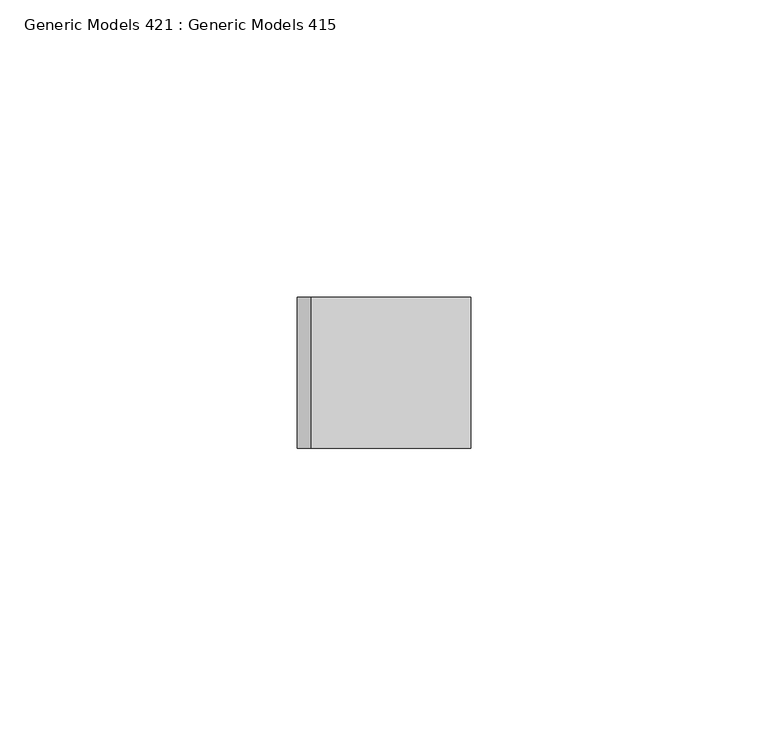
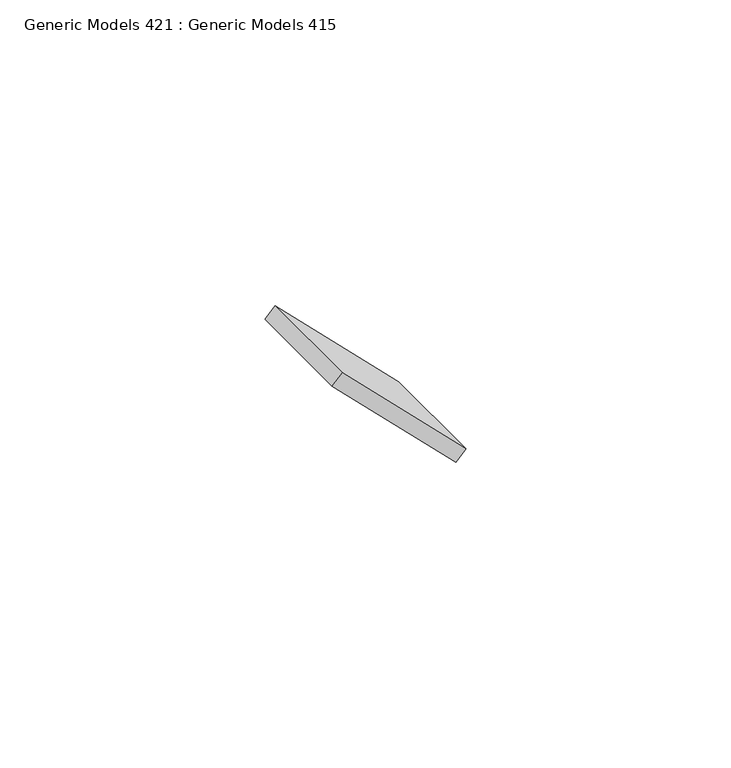
"""IFC4 building model written with IfcOpenShell, lengths in millimetres: proxy geometry, Generic Models 421 : Generic Models 415."""

from ifc_helpers import new_model, si_unit, frame, origin, place, context, project, spatial, polyline, outline, extrude, source, transform, mapped, element, save


def generic_models_421_generic_models_415_342b8473(model_context):
    return source(origin(), model_context, "Body", "SweptSolid", [
        extrude(outline(polyline([(0.0, -38.1), (0.0, 0.0), (25.4, 0.0), (25.4, -38.1), (0.0, -38.1)])), frame((-6869.8996186, -4475.9863946, 128607.0002957), z_axis=(0.7071067811864907, 0.0, 0.7071067811866044), x_axis=(0.0, -1.0, 0.0)), (0.0, 0.0, 1.0), 3.175),
    ])


if __name__ == "__main__":
    model = new_model("IFC4")
    model_context = context("Model", 3, world=origin())
    ifc_project = project(units=[si_unit("LENGTHUNIT", "METRE", prefix="MILLI")], contexts=[model_context])
    site = spatial("IfcSite", under=ifc_project)
    building = spatial("IfcBuilding", under=site)
    placement = place(None, origin())
    generic_models_421_generic_models_415_shape = generic_models_421_generic_models_415_342b8473(model_context)
    element("IfcBuildingElementProxy", 1, Name="Generic Models 421 : Generic Models 415", ObjectType="Generic Models 421 : Generic Models 415", at=placement, inside=building, context=model_context, shape_type="MappedRepresentation", body=[
        mapped(generic_models_421_generic_models_415_shape, transform((0.0, 0.0, 0.0), x_axis=(1.0, 0.0, 0.0), y_axis=(0.0, 1.0, 0.0), z_axis=(0.0, 0.0, 1.0))),
    ])
    save(model, "model.ifc")

# Revit data of these elements
# Element 1 (IfcBuildingElementProxy, "Generic Models 421 : Generic Models 415")
#   Materials on its faces: "_WELDED STEEL TABS FOR LOUVER ATTACHMENT"
# Materials
#   "_WELDED STEEL TABS FOR LOUVER ATTACHMENT": class "Metal", colour RGB 199 199 199, transparency 0, Description = "Structural steel 50ksi", Cost = 0
